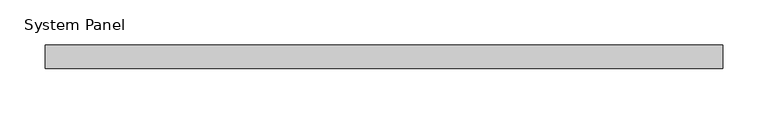
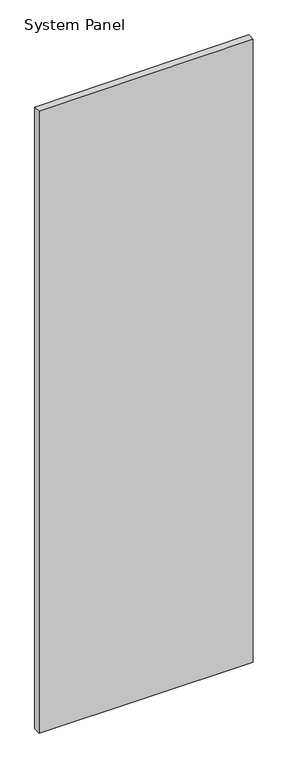
"""IFC4 building model written with IfcOpenShell, lengths in millimetres: plate geometry, System Panel : TEMPERED INSULATED GLAZING (CARDINAL GLASS LoĒ²-240."""

from ifc_helpers import new_model, si_unit, frame, origin, place, context, project, spatial, polyline, outline, extrude, source, transform, mapped, element, save


def system_panel_2a053d64(model_context):
    return source(origin(), model_context, "Body", "SweptSolid", [
        extrude(outline(polyline([(0.0, -372.4119325), (0.0, 372.4119325), (2287.5080968, 372.4119325), (2288.6997167, 372.4119325), (2283.9079061, -372.4119325), (0.0, -372.4119325)])), frame((0.0, -31.75, 0.0), z_axis=(0.0, 1.0, 0.0), x_axis=(0.0, 0.0, 1.0)), (0.0, 0.0, 1.0), 25.4),
    ])


if __name__ == "__main__":
    model = new_model("IFC4")
    model_context = context("Model", 3, world=origin())
    ifc_project = project(units=[si_unit("LENGTHUNIT", "METRE", prefix="MILLI")], contexts=[model_context])
    site = spatial("IfcSite", under=ifc_project)
    building = spatial("IfcBuilding", under=site)
    placement = place(None, origin())
    system_panel_shape = system_panel_2a053d64(model_context)
    element("IfcPlate", 1, ObjectType="System Panel : TEMPERED INSULATED GLAZING (CARDINAL GLASS LoĒ²-240", at=placement, inside=building, context=model_context, shape_type="MappedRepresentation", body=[
        mapped(system_panel_shape, transform((0.0, 0.0, 0.0), x_axis=(1.0, 0.0, 0.0), y_axis=(0.0, 1.0, 0.0), z_axis=(0.0, 0.0, 1.0))),
    ])
    save(model, "model.ifc")

# Revit data of these elements
# Type "System Panel : TEMPERED INSULATED GLAZING (CARDINAL GLASS LoĒ²-240"
#   Construction Type Id = "opn-s72"
#   Analytic Construction = "Double glazing - 1/4 in thick - low-E/clear (e = 0.1) glass"
#   Visual Light Transmittance = 0.72
#   Solar Heat Gain Coefficient = 0.6
#   Heat Transfer Coefficient (U) = 1.9873 W/(m²·K)
#   Transparency_Hack = 70
# Element 1 (IfcPlate, "System Panel : TEMPERED INSULATED GLAZING (CARDINAL GLASS LoĒ²-240")
#   Materials on its faces: "TEMPERED INSULATED GLAZING (CARDINAL GLASS LoĒ²-240\nOR EQUIVALENT)"
# Materials
#   "TEMPERED INSULATED GLAZING (CARDINAL GLASS LoĒ²-240\nOR EQUIVALENT)": class "Glass", colour RGB 196 205 210, transparency 0.85, Description = "Soda Lime Glass", Cost = 0
